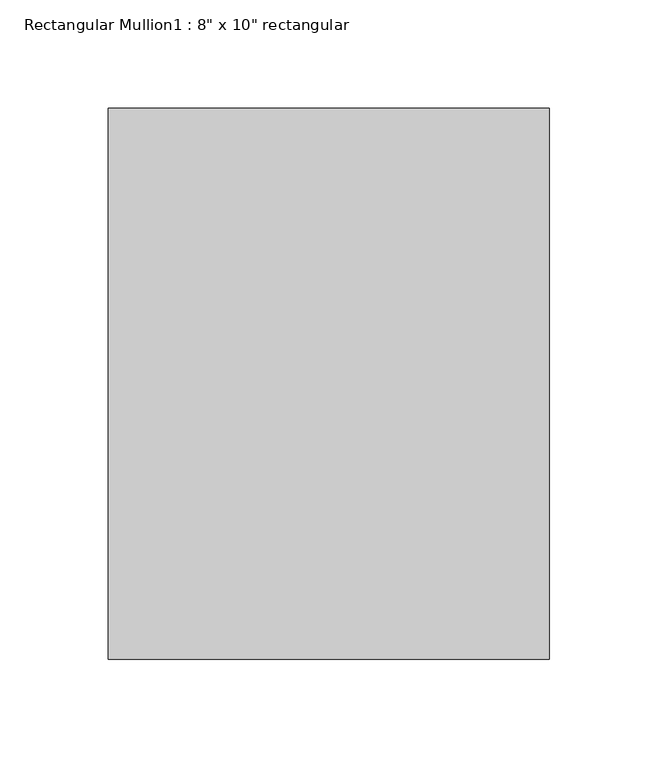
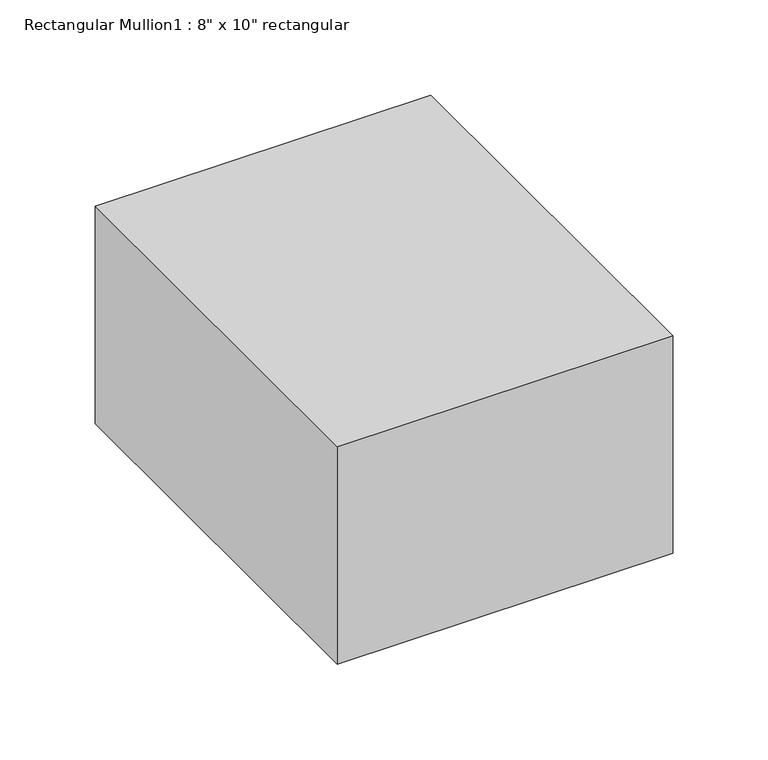
"""IFC4 building model written with IfcOpenShell, lengths in millimetres: member geometry."""

from ifc_helpers import new_model, si_unit, frame, origin, place, context, project, spatial, polyline, outline, extrude, source, transform, mapped, element, save


def member_eb4aacb2(model_context):
    return source(origin(), model_context, "Body", "SweptSolid", [
        extrude(outline(polyline([(101.6, 127.0), (101.6, -127.0), (-101.6, -127.0), (-101.6, 127.0), (101.6, 127.0)])), frame((0.0, 0.0, -139.2998379), z_axis=(0.0, 0.0, 1.0), x_axis=(1.0, 0.0, 0.0)), (0.0, 0.0, 1.0), 139.2998379),
    ])


if __name__ == "__main__":
    model = new_model("IFC4")
    model_context = context("Model", 3, world=origin())
    ifc_project = project(units=[si_unit("LENGTHUNIT", "METRE", prefix="MILLI")], contexts=[model_context])
    site = spatial("IfcSite", under=ifc_project)
    building = spatial("IfcBuilding", under=site)
    placement = place(None, origin())
    member_shape = member_eb4aacb2(model_context)
    element("IfcMember", 1, ObjectType="Rectangular Mullion1 : 8\" x 10\" rectangular", at=placement, inside=building, context=model_context, shape_type="MappedRepresentation", body=[
        mapped(member_shape, transform((0.0, 0.0, 0.0), x_axis=(1.0, 0.0, 0.0), y_axis=(0.0, 1.0, 0.0), z_axis=(0.0, 0.0, 1.0))),
    ])
    save(model, "model.ifc")

# Revit data of these elements
# Type "Rectangular Mullion1 : 8\" x 10\" rectangular"
#   built-in parameter 1007304 = 0.833333 (stored number, unit not read)
#   built-in parameter 1007301 = 0.333333 (stored number, unit not read)
#   built-in parameter 1007300 = 0.333333 (stored number, unit not read)
# Element 1 (IfcMember, "Rectangular Mullion1 : 8\" x 10\" rectangular")
#   Materials on its faces: "support-frame"
# Materials
#   "support-frame": class "Unassigned", colour RGB 233 233 233, transparency 0, Cost = 0
